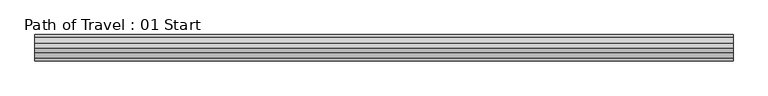
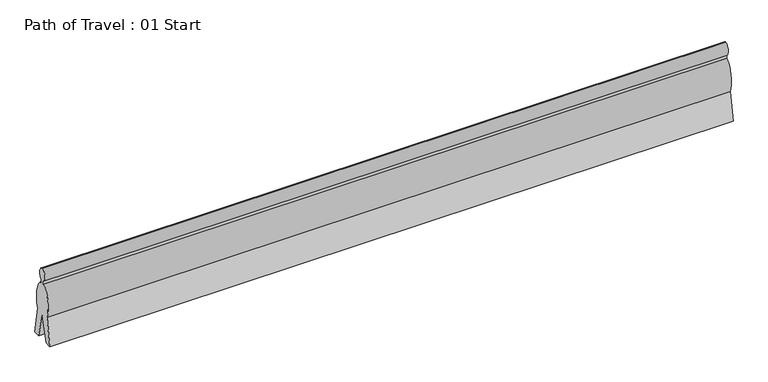
"""IFC4 building model written with IfcOpenShell, lengths in millimetres: proxy geometry, Path of Travel : 01 Start."""

from ifc_helpers import new_model, si_unit, point, frame, origin, place, context, project, spatial, ellipse_curve, trimmed, source, transform, mapped, element, save
from ifc_brep_helpers import plane_surface, extruded_surface, advanced_brep


def path_of_travel_01_start_a3c9df5a(model_context):
    return source(origin(), model_context, "Body", "AdvancedBrep", [
        advanced_brep(
        [(227.5554837, 0.0, 1727.2), (227.5554837, 42.9018657, 1436.6534209), (227.5554837, 42.9018657, 1363.4763406), (227.5554837, 184.1186263, 643.4144547), (227.5554837, 297.5699544, 0.0), (227.5554837, 145.6574193, 0.0), (227.5554837, 0.0, 584.2), (227.5554837, -145.6574193, 0.0), (227.5554837, -297.5699544, 0.0), (227.5554837, -184.1186263, 643.4144547), (227.5554837, -42.9018657, 1363.4763406), (227.5554837, -42.9018657, 1436.6534209), (15899.3554837, 0.0, 1727.2), (15899.3554837, -42.9018657, 1436.6534209), (15899.3554837, -42.9018657, 1363.4763406), (15899.3554837, -184.1186263, 643.4144547), (15899.3554837, -297.5699544, 0.0), (15899.3554837, -145.6574193, 0.0), (15899.3554837, 0.0, 584.2), (15899.3554837, 145.6574193, 0.0), (15899.3554837, 297.5699544, 0.0), (15899.3554837, 184.1186263, 643.4144547), (15899.3554837, 42.9018657, 1363.4763406), (15899.3554837, 42.9018657, 1436.6534209)],
        [
            (0, 1, ellipse_curve(frame((227.5554837, 0.0, 1574.8), z_axis=(-1.0, 0.0, 0.0), x_axis=(0.0, 0.0, 1.0)), 152.4, 101.6)),
            (1, 2),
            (2, 3, ellipse_curve(frame((227.5554837, 0.0, 914.4), z_axis=(-1.0, 0.0, 0.0), x_axis=(0.0, 0.0, -1.0)), 457.2, 228.6)),
            (3, 4),
            (4, 5),
            (5, 6),
            (6, 7),
            (7, 8),
            (8, 9),
            (9, 10, ellipse_curve(frame((227.5554837, 0.0, 914.4), z_axis=(-1.0, 0.0, 0.0), x_axis=(0.0, 0.0, -1.0)), 457.2, 228.6)),
            (10, 11),
            (11, 0, ellipse_curve(frame((227.5554837, 0.0, 1574.8), z_axis=(-1.0, 0.0, 0.0), x_axis=(0.0, 0.0, 1.0)), 152.4, 101.6)),
            (12, 13, ellipse_curve(frame((15899.3554837, 0.0, 1574.8), z_axis=(1.0, 0.0, 0.0), x_axis=(0.0, 0.0, 1.0)), 152.4, 101.6)),
            (13, 14),
            (14, 15, ellipse_curve(frame((15899.3554837, 0.0, 914.4), z_axis=(1.0, 0.0, 0.0), x_axis=(0.0, 0.0, -1.0)), 457.2, 228.6)),
            (15, 16),
            (16, 17),
            (17, 18),
            (18, 19),
            (19, 20),
            (20, 21),
            (21, 22, ellipse_curve(frame((15899.3554837, 0.0, 914.4), z_axis=(1.0, 0.0, 0.0), x_axis=(0.0, 0.0, -1.0)), 457.2, 228.6)),
            (22, 23),
            (23, 12, ellipse_curve(frame((15899.3554837, 0.0, 1574.8), z_axis=(1.0, 0.0, 0.0), x_axis=(0.0, 0.0, 1.0)), 152.4, 101.6)),
            (0, 12),
            (23, 1),
            (22, 2),
            (21, 3),
            (20, 4),
            (19, 5),
            (18, 6),
            (17, 7),
            (16, 8),
            (15, 9),
            (14, 10),
            (13, 11),
        ],
        [
            plane_surface(frame((227.5554837, 0.0, 0.0), z_axis=(-1.0, 0.0, 0.0), x_axis=(0.0, 0.0, 1.0))),
            plane_surface(frame((15899.3554837, 0.0, 0.0), z_axis=(1.0, 0.0, 0.0), x_axis=(0.0, 0.0, 1.0))),
            extruded_surface(trimmed(ellipse_curve(frame((15899.3554837, 0.0, 1574.8), z_axis=(-1.0, 0.0, 0.0), x_axis=(0.0, 0.0, 1.0)), 152.4, 101.6), [point((15899.3554837, 0.0, 1727.2))], [point((15899.3554837, 42.9018657, 1436.6534209))], True, "CARTESIAN"), (-15671.8, 0.0, 0.0), 15671.8),
            plane_surface(frame((227.5554837, 42.9018657, 1436.6534209), z_axis=(0.0, 1.0, 0.0), x_axis=(1.0, 0.0, 0.0))),
            extruded_surface(trimmed(ellipse_curve(frame((15899.3554837, 0.0, 914.4), z_axis=(-1.0, 0.0, 0.0), x_axis=(0.0, 0.0, -1.0)), 457.2, 228.6), [point((15899.3554837, 42.9018657, 1363.4763406))], [point((15899.3554837, 184.1186263, 643.4144547))], True, "CARTESIAN"), (-15671.8, 0.0, 0.0), 15671.8),
            plane_surface(frame((227.5554837, 184.1186263, 643.4144547), z_axis=(0.0, 0.9848077530122078, 0.17364817766693205), x_axis=(1.0, 0.0, 0.0))),
            plane_surface(frame((227.5554837, 297.5699544, 0.0), z_axis=(0.0, 0.0, -1.0), x_axis=(1.0, 0.0, 0.0))),
            plane_surface(frame((227.5554837, 145.6574193, 0.0), z_axis=(0.0, -0.9702957262760199, -0.2419218955995739), x_axis=(1.0, 0.0, 0.0))),
            plane_surface(frame((227.5554837, 0.0, 584.2), z_axis=(0.0, 0.9702957262759961, -0.24192189559966923), x_axis=(1.0, 0.0, 0.0))),
            plane_surface(frame((227.5554837, -145.6574193, 0.0), z_axis=(0.0, 0.0, -1.0), x_axis=(1.0, 0.0, 0.0))),
            plane_surface(frame((227.5554837, -297.5699544, 0.0), z_axis=(0.0, -0.984807753012208, 0.17364817766693066), x_axis=(1.0, 0.0, 0.0))),
            extruded_surface(trimmed(ellipse_curve(frame((15899.3554837, 0.0, 914.4), z_axis=(-1.0, 0.0, 0.0), x_axis=(0.0, 0.0, -1.0)), 457.2, 228.6), [point((15899.3554837, -184.1186263, 643.4144547))], [point((15899.3554837, -42.9018657, 1363.4763406))], True, "CARTESIAN"), (-15671.8, 0.0, 0.0), 15671.8),
            plane_surface(frame((227.5554837, -42.9018657, 1363.4763406), z_axis=(0.0, -1.0, 0.0), x_axis=(1.0, 0.0, 0.0))),
            extruded_surface(trimmed(ellipse_curve(frame((15899.3554837, 0.0, 1574.8), z_axis=(-1.0, 0.0, 0.0), x_axis=(0.0, 0.0, 1.0)), 152.4, 101.6), [point((15899.3554837, -42.9018657, 1436.6534209))], [point((15899.3554837, 0.0, 1727.2))], True, "CARTESIAN"), (-15671.8, 0.0, 0.0), 15671.8),
        ],
        [
            (0, [[1, 2, 3, 4, 5, 6, 7, 8, 9, 10, 11, 12]]),
            (1, [[13, 14, 15, 16, 17, 18, 19, 20, 21, 22, 23, 24]]),
            (2, [[-1, 25, -24, 26]]),
            (3, [[-2, -26, -23, 27]]),
            (4, [[-3, -27, -22, 28]]),
            (5, [[-4, -28, -21, 29]]),
            (6, [[-5, -29, -20, 30]]),
            (7, [[-6, -30, -19, 31]]),
            (8, [[-7, -31, -18, 32]]),
            (9, [[-8, -32, -17, 33]]),
            (10, [[-9, -33, -16, 34]]),
            (11, [[-10, -34, -15, 35]]),
            (12, [[-11, -35, -14, 36]]),
            (13, [[-12, -36, -13, -25]]),
        ],
    ),
    ])


if __name__ == "__main__":
    model = new_model("IFC4")
    model_context = context("Model", 3, world=origin())
    ifc_project = project(units=[si_unit("LENGTHUNIT", "METRE", prefix="MILLI")], contexts=[model_context])
    site = spatial("IfcSite", under=ifc_project)
    building = spatial("IfcBuilding", under=site)
    placement = place(None, origin())
    path_of_travel_01_start_shape = path_of_travel_01_start_a3c9df5a(model_context)
    element("IfcBuildingElementProxy", 1, Name="Path of Travel : 01 Start", ObjectType="Path of Travel : 01 Start", at=placement, inside=building, context=model_context, shape_type="MappedRepresentation", body=[
        mapped(path_of_travel_01_start_shape, transform((0.0, 0.0, 0.0), x_axis=(1.0, 0.0, 0.0), y_axis=(0.0, 1.0, 0.0), z_axis=(0.0, 0.0, 1.0))),
    ])
    save(model, "model.ifc")

# Revit data of these elements
# Type "Path of Travel : 01 Start"
#   Path of Egress [instance default] = 4' - 0"
#   built-in parameter 1001306 [instance default] = 4 (stored number, unit not read)
#   Dot at Start = yes
#   Arrow in Middle = yes
#   Arrow at End = no
#   Egress Path = none
# Element 1 (IfcBuildingElementProxy, "Path of Travel : 01 Start")
#   Path of Egress = 51' - 5"
#   built-in parameter 1001306 = 51.4167 (stored number, unit not read)
#   Materials on its faces: "Egress Path Solid"
# Materials
#   "Egress Path Solid": class "Unassigned", colour RGB 255 128 64, transparency 0.75, Comments = "Rendering appearance not upgraded "
